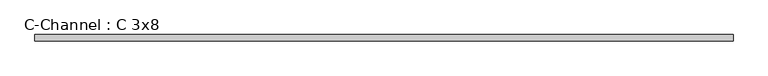
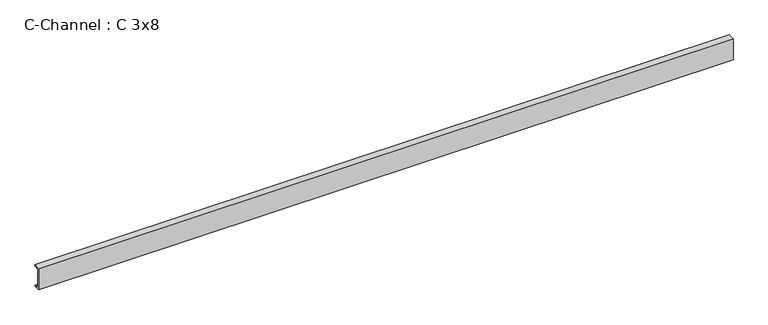
"""IFC4 building model written with IfcOpenShell, lengths in millimetres: beam geometry, C-Channel : C 3x8."""

from ifc_helpers import new_model, si_unit, point, frame, frame_2d, origin, place, context, project, spatial, polyline, circle_curve, trimmed, segment, composite_curve, outline, extrude, source, transform, mapped, element, save


def c_channel_c_3x8_649f6971(model_context):
    return source(origin(), model_context, "Body", "SweptSolid", [
        extrude(outline(composite_curve([segment(polyline([(-13.5128, 101.6), (44.9072, 101.6)]), True, "CONTINUOUS"), segment(trimmed(circle_curve(frame_2d((35.6108, 101.6)), 9.2964), [point((44.9072, 101.6))], [point((35.6108, 92.3036))], False, "CARTESIAN"), True, "CONTINUOUS"), segment(polyline([(35.6108, 92.3036), (-2.8702, 86.2088084), (-2.8702, -86.2088084), (35.6108, -92.3036)]), True, "CONTINUOUS"), segment(trimmed(circle_curve(frame_2d((35.6108, -101.6)), 9.2964), [point((35.6108, -92.3036))], [point((44.9072, -101.6))], False, "CARTESIAN"), True, "CONTINUOUS"), segment(polyline([(44.9072, -101.6), (-13.5128, -101.6), (-13.5128, 101.6)]), True, "CONTINUOUS")], self_intersect=False)), frame((-3168.65, 0.0, 0.0), z_axis=(1.0, 0.0, 0.0), x_axis=(0.0, 1.0, 0.0)), (0.0, 0.0, 1.0), 6337.3),
    ])


if __name__ == "__main__":
    model = new_model("IFC4")
    model_context = context("Model", 3, world=origin())
    ifc_project = project(units=[si_unit("LENGTHUNIT", "METRE", prefix="MILLI")], contexts=[model_context])
    site = spatial("IfcSite", under=ifc_project)
    building = spatial("IfcBuilding", under=site)
    placement = place(None, origin())
    c_channel_c_3x8_shape = c_channel_c_3x8_649f6971(model_context)
    element("IfcBeam", 1, ObjectType="C-Channel : C 3x8", at=placement, inside=building, context=model_context, shape_type="MappedRepresentation", body=[
        mapped(c_channel_c_3x8_shape, transform((0.0, 0.0, 0.0), x_axis=(1.0, 0.0, 0.0), y_axis=(0.0, 1.0, 0.0), z_axis=(0.0, 0.0, 1.0))),
    ])
    save(model, "model.ifc")

# Revit data of these elements
# Type "C-Channel : C 3x8"
#   Assembly Code = "B10"
#   W = 14.7
#   Length [instance default] = 5' - 0"
#   bf = 0' - 2.3"
#   d = 0' - 8"
#   tf = 0' - 0.366"
#   tw = 0' - 0.419"
#   x = 0' - 0.532"
#   A = 0.0300694 SF
#   Structural Material [instance default] = Steel ASTM A36
# Element 1 (IfcBeam, "C-Channel : C 3x8")
#   Structural Material = Steel ASTM A992
#   Materials on its faces: "Steel ASTM A992"
# Materials
#   "Steel ASTM A36": class "Metal", colour RGB 199 199 199, transparency 0, Description = "Structural steel, ASTM A36 Grade B, mill finish", Cost = 0
#   "Steel ASTM A992": class "Metal", colour RGB 189 187 185, transparency 0, Description = "Structural steel 50ksi", Cost = 0
